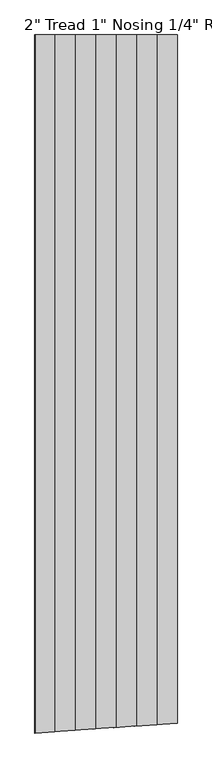
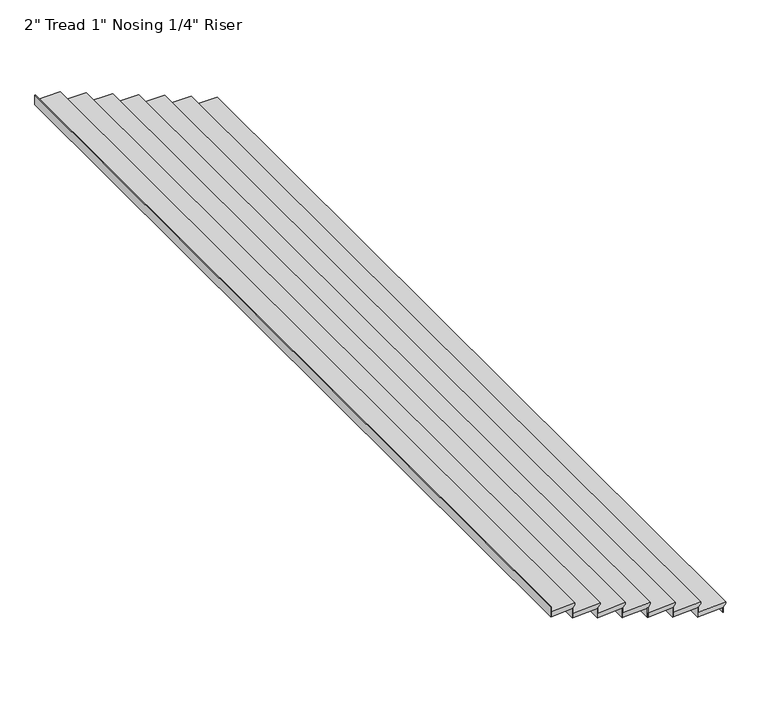
"""IFC4 building model written with IfcOpenShell, lengths in millimetres: stair flight geometry."""

from ifc_helpers import new_model, si_unit, origin, place, context, project, spatial, faceted_brep, source, transform, mapped, element, save


def stair_flight_5cbbd5cd(model_context):
    return source(origin(), model_context, "Body", "Brep", [
        faceted_brep([(13780.6252384, -2446.2319712, 1799.4474874), (13780.6252384, -2446.2319712, 1818.4974874), (13780.6252384, -11837.0822017, 1818.4974874), (13780.6252384, -11837.0822017, 1799.4474874), (13755.2252384, -2446.2319712, 1774.0474874), (13755.2252384, -11838.8583427, 1774.0474874), (13475.8252384, -2446.2319712, 1818.4974874), (13475.8252384, -11858.395894, 1818.4974874), (13755.2252384, -11838.8583427, 1767.6974874), (13475.8252384, -11858.395894, 1767.6974874), (13475.8252384, -2446.2319712, 1767.6974874), (13755.2252384, -2446.2319712, 1767.6974874)], [[[0, 1, 2, 3]], [[4, 0, 3, 5]], [[2, 1, 6, 7]], [[8, 9, 10, 11]], [[2, 7, 9, 8, 5, 3]], [[8, 11, 4, 5]], [[6, 1, 0, 4, 11, 10]], [[7, 6, 10, 9]]]),
        faceted_brep([(13755.2252384, -2446.2319712, 1767.6974874), (13755.2252384, -2446.2319712, 1710.9974874), (13748.8752384, -2446.2319712, 1710.9974874), (13748.8752384, -2446.2319712, 1767.6974874), (13755.2252384, -11838.8583427, 1767.6974874), (13748.8752384, -11839.302378, 1767.6974874), (13748.8752384, -11839.302378, 1710.9974874), (13755.2252384, -11838.8583427, 1710.9974874)], [[[0, 1, 2, 3]], [[4, 5, 6, 7]], [[1, 0, 4, 7]], [[2, 1, 7, 6]], [[3, 2, 6, 5]], [[0, 3, 5, 4]]]),
        faceted_brep([(13475.8252384, -2446.2319712, 1875.1974874), (13475.8252384, -2446.2319712, 1767.6974874), (13469.4752384, -2446.2319712, 1767.6974874), (13469.4752384, -2446.2319712, 1875.1974874), (13475.8252384, -11858.395894, 1875.1974874), (13469.4752384, -11858.8399293, 1875.1974874), (13469.4752384, -11858.8399293, 1767.6974874), (13475.8252384, -11858.395894, 1767.6974874)], [[[0, 1, 2, 3]], [[4, 5, 6, 7]], [[1, 0, 4, 7]], [[2, 1, 7, 6]], [[3, 2, 6, 5]], [[0, 3, 5, 4]]]),
        faceted_brep([(13501.2252384, -11856.619753, 1925.9974874), (13501.2252384, -2446.2319712, 1925.9974874), (13196.4252384, -2446.2319712, 1925.9974874), (13196.4252384, -11877.9334453, 1925.9974874), (13475.8252384, -11858.395894, 1875.1974874), (13196.4252384, -11877.9334453, 1875.1974874), (13196.4252384, -2446.2319712, 1875.1974874), (13475.8252384, -2446.2319712, 1875.1974874), (13475.8252384, -11858.395894, 1881.5474874), (13501.2252384, -11856.619753, 1906.9474874), (13475.8252384, -2446.2319712, 1881.5474874), (13501.2252384, -2446.2319712, 1906.9474874)], [[[0, 1, 2, 3]], [[4, 5, 6, 7]], [[0, 3, 5, 4, 8, 9]], [[4, 7, 10, 8]], [[2, 1, 11, 10, 7, 6]], [[3, 2, 6, 5]], [[11, 1, 0, 9]], [[10, 11, 9, 8]]]),
        faceted_brep([(11841.1374862, -2446.2319712, 2520.1974874), (11841.1374862, -2446.2319712, 2412.6974874), (11834.7874862, -2446.2319712, 2412.6974874), (11834.7874862, -2446.2319712, 2520.1974874), (11841.1374862, -11972.704397, 2520.1974874), (11834.7874862, -11973.1484323, 2520.1974874), (11834.7874862, -11973.1484323, 2412.6974874), (11841.1374862, -11972.704397, 2412.6974874)], [[[0, 1, 2, 3]], [[4, 5, 6, 7]], [[1, 0, 4, 7]], [[2, 1, 7, 6]], [[3, 2, 6, 5]], [[0, 3, 5, 4]]]),
        faceted_brep([(13196.4252384, -2446.2319712, 1982.6974874), (13196.4252384, -2446.2319712, 1875.1974874), (13190.0752384, -2446.2319712, 1875.1974874), (13190.0752384, -2446.2319712, 1982.6974874), (13196.4252384, -11877.9334453, 1982.6974874), (13190.0752384, -11878.3774805, 1982.6974874), (13190.0752384, -11878.3774805, 1875.1974874), (13196.4252384, -11877.9334453, 1875.1974874)], [[[0, 1, 2, 3]], [[4, 5, 6, 7]], [[1, 0, 4, 7]], [[2, 1, 7, 6]], [[3, 2, 6, 5]], [[0, 3, 5, 4]]]),
        faceted_brep([(13221.8252384, -11876.1573042, 2033.4974874), (13221.8252384, -2446.2319712, 2033.4974874), (12917.0252384, -2446.2319712, 2033.4974874), (12917.0252384, -11897.4709965, 2033.4974874), (13196.4252384, -11877.9334453, 1982.6974874), (12917.0252384, -11897.4709965, 1982.6974874), (12917.0252384, -2446.2319712, 1982.6974874), (13196.4252384, -2446.2319712, 1982.6974874), (13196.4252384, -11877.9334453, 1989.0474874), (13221.8252384, -11876.1573042, 2014.4474874), (13196.4252384, -2446.2319712, 1989.0474874), (13221.8252384, -2446.2319712, 2014.4474874)], [[[0, 1, 2, 3]], [[4, 5, 6, 7]], [[0, 3, 5, 4, 8, 9]], [[4, 7, 10, 8]], [[2, 1, 11, 10, 7, 6]], [[3, 2, 6, 5]], [[11, 1, 0, 9]], [[10, 11, 9, 8]]]),
        faceted_brep([(12917.0252384, -2446.2319712, 2090.1974874), (12917.0252384, -2446.2319712, 1982.6974874), (12910.6752384, -2446.2319712, 1982.6974874), (12910.6752384, -2446.2319712, 2090.1974874), (12917.0252384, -11897.4709965, 2090.1974874), (12910.6752384, -11897.9150318, 2090.1974874), (12910.6752384, -11897.9150318, 1982.6974874), (12917.0252384, -11897.4709965, 1982.6974874)], [[[0, 1, 2, 3]], [[4, 5, 6, 7]], [[1, 0, 4, 7]], [[2, 1, 7, 6]], [[3, 2, 6, 5]], [[0, 3, 5, 4]]]),
        faceted_brep([(12942.4252384, -11895.6948555, 2140.9974874), (12942.4252384, -2446.2319712, 2140.9974874), (12637.6252384, -2446.2319712, 2140.9974874), (12637.6252384, -11917.0085478, 2140.9974874), (12917.0252384, -11897.4709965, 2090.1974874), (12637.6252384, -11917.0085478, 2090.1974874), (12637.6252384, -2446.2319712, 2090.1974874), (12917.0252384, -2446.2319712, 2090.1974874), (12917.0252384, -11897.4709965, 2096.5474874), (12942.4252384, -11895.6948555, 2121.9474874), (12917.0252384, -2446.2319712, 2096.5474874), (12942.4252384, -2446.2319712, 2121.9474874)], [[[0, 1, 2, 3]], [[4, 5, 6, 7]], [[0, 3, 5, 4, 8, 9]], [[4, 7, 10, 8]], [[2, 1, 11, 10, 7, 6]], [[3, 2, 6, 5]], [[11, 1, 0, 9]], [[10, 11, 9, 8]]]),
        faceted_brep([(12637.6252384, -2446.2319712, 2197.6974874), (12637.6252384, -2446.2319712, 2090.1974874), (12631.2752384, -2446.2319712, 2090.1974874), (12631.2752384, -2446.2319712, 2197.6974874), (12637.6252384, -11917.0085478, 2197.6974874), (12631.2752384, -11917.452583, 2197.6974874), (12631.2752384, -11917.452583, 2090.1974874), (12637.6252384, -11917.0085478, 2090.1974874)], [[[0, 1, 2, 3]], [[4, 5, 6, 7]], [[1, 0, 4, 7]], [[2, 1, 7, 6]], [[3, 2, 6, 5]], [[0, 3, 5, 4]]]),
        faceted_brep([(12663.0252384, -11915.2324067, 2248.4974874), (12663.0252384, -2446.2319712, 2248.4974874), (12358.2252384, -2446.2319712, 2248.4974874), (12358.2252384, -11936.546099, 2248.4974874), (12637.6252384, -11917.0085478, 2197.6974874), (12358.2252384, -11936.546099, 2197.6974874), (12358.2252384, -2446.2319712, 2197.6974874), (12637.6252384, -2446.2319712, 2197.6974874), (12637.6252384, -11917.0085478, 2204.0474874), (12663.0252384, -11915.2324067, 2229.4474874), (12637.6252384, -2446.2319712, 2204.0474874), (12663.0252384, -2446.2319712, 2229.4474874)], [[[0, 1, 2, 3]], [[4, 5, 6, 7]], [[0, 3, 5, 4, 8, 9]], [[4, 7, 10, 8]], [[2, 1, 11, 10, 7, 6]], [[3, 2, 6, 5]], [[11, 1, 0, 9]], [[10, 11, 9, 8]]]),
        faceted_brep([(12358.2252384, -2446.2319712, 2305.1974874), (12358.2252384, -2446.2319712, 2197.6974874), (12351.8752384, -2446.2319712, 2197.6974874), (12351.8752384, -2446.2319712, 2305.1974874), (12358.2252384, -11936.546099, 2305.1974874), (12351.8752384, -11936.9901343, 2305.1974874), (12351.8752384, -11936.9901343, 2197.6974874), (12358.2252384, -11936.546099, 2197.6974874)], [[[0, 1, 2, 3]], [[4, 5, 6, 7]], [[1, 0, 4, 7]], [[2, 1, 7, 6]], [[3, 2, 6, 5]], [[0, 3, 5, 4]]]),
        faceted_brep([(12383.6252384, -11934.769958, 2355.9974874), (12383.6252384, -2446.2319712, 2355.9974874), (12078.8252384, -2446.2319712, 2355.9974874), (12078.8252384, -11956.0836503, 2355.9974874), (12358.2252384, -11936.546099, 2305.1974874), (12078.8252384, -11956.0836503, 2305.1974874), (12078.8252384, -2446.2319712, 2305.1974874), (12358.2252384, -2446.2319712, 2305.1974874), (12358.2252384, -11936.546099, 2311.5474874), (12383.6252384, -11934.769958, 2336.9474874), (12358.2252384, -2446.2319712, 2311.5474874), (12383.6252384, -2446.2319712, 2336.9474874)], [[[0, 1, 2, 3]], [[4, 5, 6, 7]], [[0, 3, 5, 4, 8, 9]], [[4, 7, 10, 8]], [[2, 1, 11, 10, 7, 6]], [[3, 2, 6, 5]], [[11, 1, 0, 9]], [[10, 11, 9, 8]]]),
        faceted_brep([(12078.8252384, -2446.2319712, 2412.6974874), (12078.8252384, -2446.2319712, 2305.1974874), (12072.4752384, -2446.2319712, 2305.1974874), (12072.4752384, -2446.2319712, 2412.6974874), (12078.8252384, -11956.0836503, 2412.6974874), (12072.4752384, -11956.5276855, 2412.6974874), (12072.4752384, -11956.5276855, 2305.1974874), (12078.8252384, -11956.0836503, 2305.1974874)], [[[0, 1, 2, 3]], [[4, 5, 6, 7]], [[1, 0, 4, 7]], [[2, 1, 7, 6]], [[3, 2, 6, 5]], [[0, 3, 5, 4]]]),
        faceted_brep([(12104.2252384, -11954.3075093, 2463.4974874), (12104.2252384, -2446.2319712, 2463.4974874), (11841.1374862, -2446.2319712, 2463.4974874), (11841.1374862, -11972.704397, 2463.4974874), (12078.8252384, -11956.0836503, 2412.6974874), (11841.1374862, -11972.704397, 2412.6974874), (11841.1374862, -2446.2319712, 2412.6974874), (12078.8252384, -2446.2319712, 2412.6974874), (12078.8252384, -11956.0836503, 2419.0474874), (12104.2252384, -11954.3075093, 2444.4474874), (12078.8252384, -2446.2319712, 2419.0474874), (12104.2252384, -2446.2319712, 2444.4474874)], [[[0, 1, 2, 3]], [[4, 5, 6, 7]], [[0, 3, 5, 4, 8, 9]], [[4, 7, 10, 8]], [[2, 1, 11, 10, 7, 6]], [[3, 2, 6, 5]], [[11, 1, 0, 9]], [[10, 11, 9, 8]]]),
    ])


if __name__ == "__main__":
    model = new_model("IFC4")
    model_context = context("Model", 3, world=origin())
    ifc_project = project(units=[si_unit("LENGTHUNIT", "METRE", prefix="MILLI")], contexts=[model_context])
    site = spatial("IfcSite", under=ifc_project)
    building = spatial("IfcBuilding", under=site)
    placement = place(None, origin())
    stair_flight_shape = stair_flight_5cbbd5cd(model_context)
    element("IfcStairFlight", 1, ObjectType="2\" Tread 1\" Nosing 1/4\" Riser", at=placement, inside=building, context=model_context, shape_type="MappedRepresentation", body=[
        mapped(stair_flight_shape, transform((0.0, 0.0, 0.0), x_axis=(1.0, 0.0, 0.0), y_axis=(0.0, 1.0, 0.0), z_axis=(0.0, 0.0, 1.0))),
    ])
    save(model, "model.ifc")

# Revit data of these elements
# Project information
#   Project Issue Date = "Issue Date"
#   Project Status = "Project Status"
#   Client Name = "Owner"
#   Project Address = "Enter address here"
#   Project Name = "Project Name"
#   Project Number = "Project Number"
